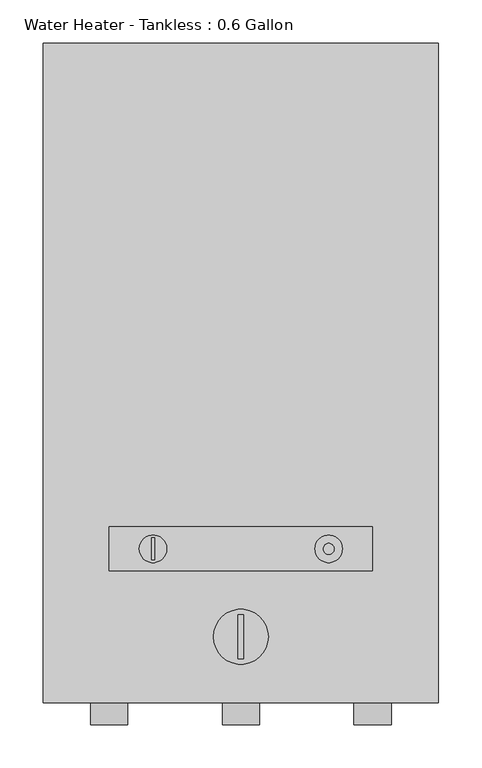
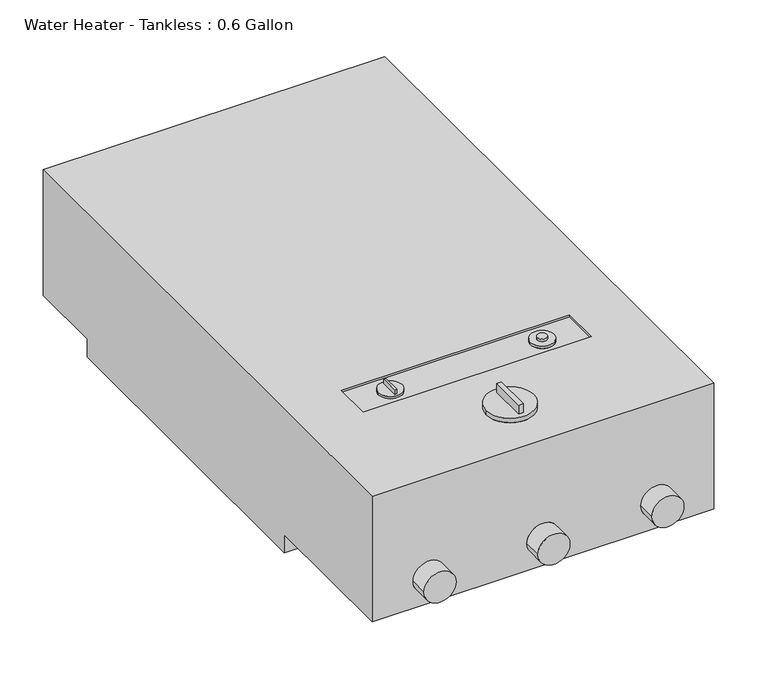
"""IFC4 building model written with IfcOpenShell, lengths in millimetres: proxy geometry, Water Heater - Tankless : 0.6 Gallon."""

from ifc_helpers import new_model, si_unit, point, frame, frame_2d, origin, place, context, project, spatial, circle_curve, trimmed, segment, composite_curve, outline, extrude, source, transform, mapped, element, save
from ifc_brep_helpers import plane_surface, cylinder_surface, advanced_brep


def water_heater_tankless_0_6_gallon_c20ab9af(model_context):
    return source(origin(), model_context, "Body", "SolidModel", [
        advanced_brep(
        [(228.6, 762.0, 25.4), (228.6, 762.0, 203.2), (228.6, 0.0, 203.2), (228.6, 0.0, 25.4), (228.6, 203.2, 25.4), (228.6, 203.2, 0.0), (228.6, 660.4, 0.0), (228.6, 660.4, 25.4), (-228.6, 762.0, 25.4), (-228.6, 660.4, 25.4), (-228.6, 660.4, 0.0), (-228.6, 203.2, 0.0), (-228.6, 203.2, 25.4), (-228.6, 0.0, 25.4), (-228.6, 0.0, 203.2), (-228.6, 762.0, 203.2), (-152.4, 203.2, 203.2), (152.4, 203.2, 203.2), (152.4, 152.4, 203.2), (-152.4, 152.4, 203.2), (31.75, 76.2, 203.2), (-31.75, 76.2, 203.2), (-130.96875, 0.0, 63.5), (-173.83125, 0.0, 63.5), (21.43125, 0.0, 63.5), (-21.43125, 0.0, 63.5), (173.83125, 0.0, 63.5), (130.96875, 0.0, 63.5), (152.4, 203.2, 200.025), (-152.4, 203.2, 200.025), (-152.4, 152.4, 200.025), (152.4, 152.4, 200.025), (-85.725, 177.8, 200.025), (-117.475, 177.8, 200.025), (117.475, 177.8, 200.025), (85.725, 177.8, 200.025), (-173.83125, -25.4, 63.5), (-130.96875, -25.4, 63.5), (-21.43125, -25.4, 63.5), (21.43125, -25.4, 63.5), (130.96875, -25.4, 63.5), (173.83125, -25.4, 63.5), (-117.475, 177.8, 203.2), (-85.725, 177.8, 203.2), (-103.1875, 190.5, 203.2), (-100.0125, 190.5, 203.2), (-100.0125, 165.1, 203.2), (-103.1875, 165.1, 203.2), (85.725, 177.8, 203.2), (117.475, 177.8, 203.2), (107.95, 177.8, 203.2), (95.25, 177.8, 203.2), (95.25, 177.8, 206.375), (107.95, 177.8, 206.375), (-100.0125, 190.5, 209.55), (-103.1875, 190.5, 209.55), (-103.1875, 165.1, 209.55), (-100.0125, 165.1, 209.55), (-31.75, 76.2, 209.55), (31.75, 76.2, 209.55), (-3.175, 101.6, 209.55), (3.175, 101.6, 209.55), (3.175, 50.8, 209.55), (-3.175, 50.8, 209.55), (3.175, 101.6, 222.25), (-3.175, 101.6, 222.25), (-3.175, 50.8, 222.25), (3.175, 50.8, 222.25)],
        [
            (0, 1),
            (1, 2),
            (2, 3),
            (3, 4),
            (4, 5),
            (5, 6),
            (6, 7),
            (7, 0),
            (8, 9),
            (9, 10),
            (10, 11),
            (11, 12),
            (12, 13),
            (13, 14),
            (14, 15),
            (15, 8),
            (0, 8),
            (15, 1),
            (14, 2),
            (16, 17),
            (17, 18),
            (18, 19),
            (19, 16),
            (20, 21, circle_curve(frame((0.0, 76.2, 203.2), z_axis=(0.0, 0.0, -1.0), x_axis=(1.0, 0.0, 0.0)), 31.75)),
            (21, 20, circle_curve(frame((0.0, 76.2, 203.2), z_axis=(0.0, 0.0, -1.0), x_axis=(1.0, 0.0, 0.0)), 31.75)),
            (13, 3),
            (22, 23, circle_curve(frame((-152.4, 0.0, 63.5), z_axis=(0.0, 1.0, 0.0), x_axis=(1.0, 0.0, 0.0)), 21.43125)),
            (23, 22, circle_curve(frame((-152.4, 0.0, 63.5), z_axis=(0.0, 1.0, 0.0), x_axis=(1.0, 0.0, 0.0)), 21.43125)),
            (24, 25, circle_curve(frame((0.0, 0.0, 63.5), z_axis=(0.0, 1.0, 0.0), x_axis=(1.0, 0.0, 0.0)), 21.43125)),
            (25, 24, circle_curve(frame((0.0, 0.0, 63.5), z_axis=(0.0, 1.0, 0.0), x_axis=(1.0, 0.0, 0.0)), 21.43125)),
            (26, 27, circle_curve(frame((152.4, 0.0, 63.5), z_axis=(0.0, 1.0, 0.0), x_axis=(1.0, 0.0, 0.0)), 21.43125)),
            (27, 26, circle_curve(frame((152.4, 0.0, 63.5), z_axis=(0.0, 1.0, 0.0), x_axis=(1.0, 0.0, 0.0)), 21.43125)),
            (12, 4),
            (11, 5),
            (10, 6),
            (9, 7),
            (28, 29),
            (29, 30),
            (30, 31),
            (31, 28),
            (32, 33, circle_curve(frame((-101.6, 177.8, 200.025), z_axis=(0.0, 0.0, -1.0), x_axis=(1.0, 0.0, 0.0)), 15.875)),
            (33, 32, circle_curve(frame((-101.6, 177.8, 200.025), z_axis=(0.0, 0.0, -1.0), x_axis=(1.0, 0.0, 0.0)), 15.875)),
            (34, 35, circle_curve(frame((101.6, 177.8, 200.025), z_axis=(0.0, 0.0, -1.0), x_axis=(1.0, 0.0, 0.0)), 15.875)),
            (35, 34, circle_curve(frame((101.6, 177.8, 200.025), z_axis=(0.0, 0.0, -1.0), x_axis=(1.0, 0.0, 0.0)), 15.875)),
            (28, 17),
            (16, 29),
            (19, 30),
            (18, 31),
            (36, 37, circle_curve(frame((-152.4, -25.4, 63.5), z_axis=(0.0, -1.0, 0.0), x_axis=(1.0, 0.0, 0.0)), 21.43125)),
            (37, 36, circle_curve(frame((-152.4, -25.4, 63.5), z_axis=(0.0, -1.0, 0.0), x_axis=(1.0, 0.0, 0.0)), 21.43125)),
            (38, 39, circle_curve(frame((0.0, -25.4, 63.5), z_axis=(0.0, -1.0, 0.0), x_axis=(1.0, 0.0, 0.0)), 21.43125)),
            (39, 38, circle_curve(frame((0.0, -25.4, 63.5), z_axis=(0.0, -1.0, 0.0), x_axis=(1.0, 0.0, 0.0)), 21.43125)),
            (40, 41, circle_curve(frame((152.4, -25.4, 63.5), z_axis=(0.0, -1.0, 0.0), x_axis=(1.0, 0.0, 0.0)), 21.43125)),
            (41, 40, circle_curve(frame((152.4, -25.4, 63.5), z_axis=(0.0, -1.0, 0.0), x_axis=(1.0, 0.0, 0.0)), 21.43125)),
            (36, 23),
            (22, 37),
            (38, 25),
            (24, 39),
            (40, 27),
            (26, 41),
            (42, 43, circle_curve(frame((-101.6, 177.8, 203.2), z_axis=(0.0, 0.0, 1.0), x_axis=(1.0, 0.0, 0.0)), 15.875)),
            (43, 42, circle_curve(frame((-101.6, 177.8, 203.2), z_axis=(0.0, 0.0, 1.0), x_axis=(1.0, 0.0, 0.0)), 15.875)),
            (44, 45),
            (45, 46),
            (46, 47),
            (47, 44),
            (48, 49, circle_curve(frame((101.6, 177.8, 203.2), z_axis=(0.0, 0.0, 1.0), x_axis=(1.0, 0.0, 0.0)), 15.875)),
            (49, 48, circle_curve(frame((101.6, 177.8, 203.2), z_axis=(0.0, 0.0, 1.0), x_axis=(1.0, 0.0, 0.0)), 15.875)),
            (50, 51, circle_curve(frame((101.6, 177.8, 203.2), z_axis=(0.0, 0.0, -1.0), x_axis=(1.0, 0.0, 0.0)), 6.35)),
            (51, 50, circle_curve(frame((101.6, 177.8, 203.2), z_axis=(0.0, 0.0, -1.0), x_axis=(1.0, 0.0, 0.0)), 6.35)),
            (42, 33),
            (32, 43),
            (48, 35),
            (34, 49),
            (52, 53, circle_curve(frame((101.6, 177.8, 206.375), z_axis=(0.0, 0.0, 1.0), x_axis=(1.0, 0.0, 0.0)), 6.35)),
            (53, 52, circle_curve(frame((101.6, 177.8, 206.375), z_axis=(0.0, 0.0, 1.0), x_axis=(1.0, 0.0, 0.0)), 6.35)),
            (52, 51),
            (50, 53),
            (54, 55),
            (55, 56),
            (56, 57),
            (57, 54),
            (54, 45),
            (44, 55),
            (47, 56),
            (46, 57),
            (58, 59, circle_curve(frame((0.0, 76.2, 209.55), z_axis=(0.0, 0.0, 1.0), x_axis=(1.0, 0.0, 0.0)), 31.75)),
            (59, 58, circle_curve(frame((0.0, 76.2, 209.55), z_axis=(0.0, 0.0, 1.0), x_axis=(1.0, 0.0, 0.0)), 31.75)),
            (60, 61),
            (61, 62),
            (62, 63),
            (63, 60),
            (58, 21),
            (20, 59),
            (64, 65),
            (65, 66),
            (66, 67),
            (67, 64),
            (64, 61),
            (60, 65),
            (63, 66),
            (62, 67),
        ],
        [
            plane_surface(frame((228.6, 762.0, 203.2), z_axis=(1.0, 0.0, 0.0), x_axis=(0.0, 0.0, 1.0))),
            plane_surface(frame((-228.6, 762.0, 203.2), z_axis=(-1.0, 0.0, 0.0), x_axis=(0.0, 0.0, -1.0))),
            plane_surface(frame((228.6, 762.0, 25.4), z_axis=(0.0, 1.0, 0.0), x_axis=(-1.0, 0.0, 0.0))),
            plane_surface(frame((228.6, 762.0, 203.2), z_axis=(0.0, 0.0, 1.0), x_axis=(-1.0, 0.0, 0.0))),
            plane_surface(frame((228.6, 0.0, 203.2), z_axis=(0.0, -1.0, 0.0), x_axis=(-1.0, 0.0, 0.0))),
            plane_surface(frame((228.6, 0.0, 25.4), z_axis=(0.0, 0.0, -1.0), x_axis=(-1.0, 0.0, 0.0))),
            plane_surface(frame((228.6, 203.2, 25.4), z_axis=(0.0, -1.0, 0.0), x_axis=(-1.0, 0.0, 0.0))),
            plane_surface(frame((228.6, 203.2, 0.0), z_axis=(0.0, 0.0, -1.0), x_axis=(-1.0, 0.0, 0.0))),
            plane_surface(frame((228.6, 660.4, 0.0), z_axis=(0.0, 1.0, 0.0), x_axis=(-1.0, 0.0, 0.0))),
            plane_surface(frame((228.6, 660.4, 25.4), z_axis=(0.0, 0.0, -1.0), x_axis=(-1.0, 0.0, 0.0))),
            plane_surface(frame((-152.4, 203.2, 200.025), z_axis=(0.0, 0.0, 1.0), x_axis=(1.0, 0.0, 0.0))),
            plane_surface(frame((152.4, 203.2, 203.2), z_axis=(0.0, -1.0, 0.0), x_axis=(0.0, 0.0, -1.0))),
            plane_surface(frame((-152.4, 203.2, 203.2), z_axis=(1.0, 0.0, 0.0), x_axis=(0.0, 0.0, -1.0))),
            plane_surface(frame((-152.4, 152.4, 203.2), z_axis=(0.0, 1.0, 0.0), x_axis=(0.0, 0.0, -1.0))),
            plane_surface(frame((152.4, 152.4, 203.2), z_axis=(-1.0, 0.0, 0.0), x_axis=(0.0, 0.0, -1.0))),
            plane_surface(frame((-130.96875, -25.4, 63.5), z_axis=(0.0, -1.0, 0.0), x_axis=(0.0, 0.0, 1.0))),
            cylinder_surface(frame((-152.4, 0.0, 63.5), z_axis=(0.0, -1.0, 0.0), x_axis=(1.0, 0.0, 0.0)), 21.43125),
            cylinder_surface(frame((0.0, 0.0, 63.5), z_axis=(0.0, -1.0, 0.0), x_axis=(1.0, 0.0, 0.0)), 21.43125),
            cylinder_surface(frame((152.4, 0.0, 63.5), z_axis=(0.0, -1.0, 0.0), x_axis=(1.0, 0.0, 0.0)), 21.43125),
            plane_surface(frame((-85.725, 177.8, 203.2), z_axis=(0.0, 0.0, 1.0), x_axis=(0.0, 1.0, 0.0))),
            cylinder_surface(frame((-101.6, 177.8, 200.025), z_axis=(0.0, 0.0, 1.0), x_axis=(1.0, 0.0, 0.0)), 15.875),
            cylinder_surface(frame((101.6, 177.8, 0.0), z_axis=(0.0, 0.0, 1.0), x_axis=(1.0, 0.0, 0.0)), 15.875),
            plane_surface(frame((107.95, 177.8, 206.375), z_axis=(0.0, 0.0, 1.0), x_axis=(0.0, 1.0, 0.0))),
            cylinder_surface(frame((101.6, 177.8, 203.2), z_axis=(0.0, 0.0, 1.0), x_axis=(1.0, 0.0, 0.0)), 6.35),
            plane_surface(frame((-103.1875, 190.5, 209.55), z_axis=(0.0, 0.0, 1.0), x_axis=(-1.0, 0.0, 0.0))),
            plane_surface(frame((-100.0125, 190.5, 209.55), z_axis=(0.0, 1.0, 0.0), x_axis=(0.0, 0.0, -1.0))),
            plane_surface(frame((-103.1875, 190.5, 209.55), z_axis=(-1.0, 0.0, 0.0), x_axis=(0.0, 0.0, -1.0))),
            plane_surface(frame((-103.1875, 165.1, 209.55), z_axis=(0.0, -1.0, 0.0), x_axis=(0.0, 0.0, -1.0))),
            plane_surface(frame((-100.0125, 165.1, 209.55), z_axis=(1.0, 0.0, 0.0), x_axis=(0.0, 0.0, -1.0))),
            plane_surface(frame((31.75, 76.2, 209.55), z_axis=(0.0, 0.0, 1.0), x_axis=(0.0, 1.0, 0.0))),
            cylinder_surface(frame((0.0, 76.2, 203.2), z_axis=(0.0, 0.0, 1.0), x_axis=(1.0, 0.0, 0.0)), 31.75),
            plane_surface(frame((-3.175, 101.6, 222.25), z_axis=(0.0, 0.0, 1.0), x_axis=(-1.0, 0.0, 0.0))),
            plane_surface(frame((3.175, 101.6, 222.25), z_axis=(0.0, 1.0, 0.0), x_axis=(0.0, 0.0, -1.0))),
            plane_surface(frame((-3.175, 101.6, 222.25), z_axis=(-1.0, 0.0, 0.0), x_axis=(0.0, 0.0, -1.0))),
            plane_surface(frame((-3.175, 50.8, 222.25), z_axis=(0.0, -1.0, 0.0), x_axis=(0.0, 0.0, -1.0))),
            plane_surface(frame((3.175, 50.8, 222.25), z_axis=(1.0, 0.0, 0.0), x_axis=(0.0, 0.0, -1.0))),
        ],
        [
            (0, [[1, 2, 3, 4, 5, 6, 7, 8]]),
            (1, [[9, 10, 11, 12, 13, 14, 15, 16]]),
            (2, [[-1, 17, -16, 18]]),
            (3, [[-2, -18, -15, 19], [20, 21, 22, 23], [24, 25]]),
            (4, [[-3, -19, -14, 26], [27, 28], [29, 30], [31, 32]]),
            (5, [[-4, -26, -13, 33]]),
            (6, [[-5, -33, -12, 34]]),
            (7, [[-6, -34, -11, 35]]),
            (8, [[-7, -35, -10, 36]]),
            (9, [[-8, -36, -9, -17]]),
            (10, [[37, 38, 39, 40], [41, 42], [43, 44]]),
            (11, [[-37, 45, -20, 46]]),
            (12, [[-38, -46, -23, 47]]),
            (13, [[-39, -47, -22, 48]]),
            (14, [[-40, -48, -21, -45]]),
            (15, [[49, 50]]),
            (15, [[51, 52]]),
            (15, [[53, 54]]),
            (16, [[-49, 55, -27, 56]]),
            (16, [[-50, -56, -28, -55]]),
            (17, [[-51, 57, -29, 58]]),
            (17, [[-52, -58, -30, -57]]),
            (18, [[-53, 59, -31, 60]]),
            (18, [[-54, -60, -32, -59]]),
            (19, [[61, 62], [63, 64, 65, 66]]),
            (19, [[67, 68], [69, 70]]),
            (20, [[-61, 71, -41, 72]]),
            (20, [[-62, -72, -42, -71]]),
            (21, [[-67, 73, -43, 74]]),
            (21, [[-68, -74, -44, -73]]),
            (22, [[75, 76]]),
            (23, [[-75, 77, -69, 78]]),
            (23, [[-76, -78, -70, -77]]),
            (24, [[79, 80, 81, 82]]),
            (25, [[-79, 83, -63, 84]]),
            (26, [[-80, -84, -66, 85]]),
            (27, [[-81, -85, -65, 86]]),
            (28, [[-82, -86, -64, -83]]),
            (29, [[87, 88], [89, 90, 91, 92]]),
            (30, [[-87, 93, -24, 94]]),
            (30, [[-88, -94, -25, -93]]),
            (31, [[95, 96, 97, 98]]),
            (32, [[-95, 99, -89, 100]]),
            (33, [[-96, -100, -92, 101]]),
            (34, [[-97, -101, -91, 102]]),
            (35, [[-98, -102, -90, -99]]),
        ],
    ),
        extrude(outline(composite_curve([segment(trimmed(circle_curve(frame_2d((0.0, 152.4)), 3.175), [point((-3.175, 152.4))], [point((3.175, 152.4))], False, "CARTESIAN"), True, "CONTINUOUS"), segment(trimmed(circle_curve(frame_2d((0.0, 152.4)), 3.175), [point((3.175, 152.4))], [point((-3.175, 152.4))], False, "CARTESIAN"), True, "CONTINUOUS")], self_intersect=False)), frame((0.0, 0.0, 25.4), z_axis=(0.0, 0.0, 1.0), x_axis=(1.0, 0.0, 0.0)), (0.0, 0.0, 1.0), 38.1),
    ])


if __name__ == "__main__":
    model = new_model("IFC4")
    model_context = context("Model", 3, world=origin())
    ifc_project = project(units=[si_unit("LENGTHUNIT", "METRE", prefix="MILLI")], contexts=[model_context])
    site = spatial("IfcSite", under=ifc_project)
    building = spatial("IfcBuilding", under=site)
    placement = place(None, origin())
    water_heater_tankless_0_6_gallon_shape = water_heater_tankless_0_6_gallon_c20ab9af(model_context)
    element("IfcBuildingElementProxy", 1, Name="Water Heater - Tankless : 0.6 Gallon", ObjectType="Water Heater - Tankless : 0.6 Gallon", at=placement, inside=building, context=model_context, shape_type="MappedRepresentation", body=[
        mapped(water_heater_tankless_0_6_gallon_shape, transform((0.0, 0.0, 0.0), x_axis=(1.0, 0.0, 0.0), y_axis=(0.0, 1.0, 0.0), z_axis=(0.0, 0.0, 1.0))),
    ])
    save(model, "model.ifc")

# Revit data of these elements
# Type "Water Heater - Tankless : 0.6 Gallon"
#   Water Heater Width = 0' - 8"
#   Water Heater Length = 1' - 6"
#   Water Heater Height = 2' - 6"
#   Voltage = 120 V
#   Vent Radius = 2"
#   Vent Diameter = 4"
#   Hot Water Radius = 1/2"
#   Hot Water Diameter = 1"
#   Half Water Heater Length = 0' - 9"
#   Gas Radius = 3/8"
#   Gas Diameter = 3/4"
#   Flow Pressure [instance default] = 25.00 psi
#   Flow [instance default] = 13 GPM
#   Default Elevation = 5' - 0"
#   Cold Water Radius = 1/2"
#   Cold Water Diameter = 1"
#   Apparent Load = 125 VA
#   Number of Poles = 1
#   Water Heater Material = none
#   Load Classification = Appliance - Dwelling Unit
# Element 1 (IfcBuildingElementProxy, "Water Heater - Tankless : 0.6 Gallon")
#   Flow = 0 GPM
